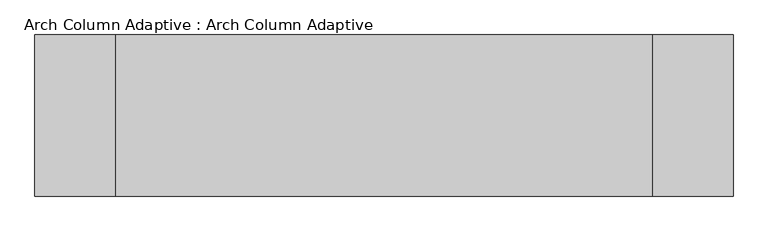
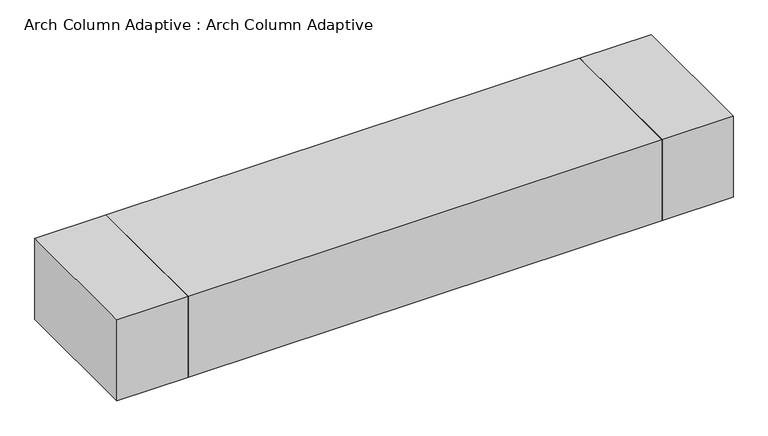
"""IFC4 building model written with IfcOpenShell, lengths in millimetres: proxy geometry, Arch Column Adaptive : Arch Column Adaptive."""

from ifc_helpers import new_model, si_unit, frame, origin, place, context, project, spatial, polyline, outline, extrude, source, transform, mapped, element, save


def arch_column_adaptive_arch_column_adaptive_6b0f74e0(model_context):
    return source(origin(), model_context, "Body", "SweptSolid", [
        extrude(outline(polyline([(5000.0, -1500.0), (5000.0, 1500.0), (6500.0, 1500.0), (6500.0, -1500.0), (5000.0, -1500.0)])), frame((0.0, 0.0, 83080.0), z_axis=(0.0, 0.0, 1.0), x_axis=(1.0, 0.0, 0.0)), (0.0, 0.0, 1.0), 1800.0),
        extrude(outline(polyline([(-5000.0, 1500.0), (-5000.0, -1500.0), (-6500.0, -1500.0), (-6500.0, 1500.0), (-5000.0, 1500.0)])), frame((0.0, 0.0, 83080.0), z_axis=(0.0, 0.0, 1.0), x_axis=(1.0, 0.0, 0.0)), (0.0, 0.0, 1.0), 1800.0),
        extrude(outline(polyline([(-5000.0, -1500.0), (-5000.0, 1500.0), (5000.0, 1500.0), (5000.0, -1500.0), (-5000.0, -1500.0)])), frame((0.0, 0.0, 83080.0), z_axis=(0.0, 0.0, 1.0), x_axis=(1.0, 0.0, 0.0)), (0.0, 0.0, 1.0), 1800.0),
    ])


if __name__ == "__main__":
    model = new_model("IFC4")
    model_context = context("Model", 3, world=origin())
    ifc_project = project(units=[si_unit("LENGTHUNIT", "METRE", prefix="MILLI")], contexts=[model_context])
    site = spatial("IfcSite", under=ifc_project)
    building = spatial("IfcBuilding", under=site)
    placement = place(None, origin())
    arch_column_adaptive_arch_column_adaptive_shape = arch_column_adaptive_arch_column_adaptive_6b0f74e0(model_context)
    element("IfcBuildingElementProxy", 1, Name="Arch Column Adaptive : Arch Column Adaptive", ObjectType="Arch Column Adaptive : Arch Column Adaptive", at=placement, inside=building, context=model_context, shape_type="MappedRepresentation", body=[
        mapped(arch_column_adaptive_arch_column_adaptive_shape, transform((0.0, 0.0, 0.0), x_axis=(1.0, 0.0, 0.0), y_axis=(0.0, 1.0, 0.0), z_axis=(0.0, 0.0, 1.0))),
    ])
    save(model, "model.ifc")

# Revit data of these elements
# Type "Arch Column Adaptive : Arch Column Adaptive"
#   Top Width = 3000 mm
#   Length [instance default] = 21000 mm
#   Height [instance default] = 50000 mm
#   Default Elevation = 0
# Element 1 (IfcBuildingElementProxy, "Arch Column Adaptive : Arch Column Adaptive")
#   Height = 83080 mm
